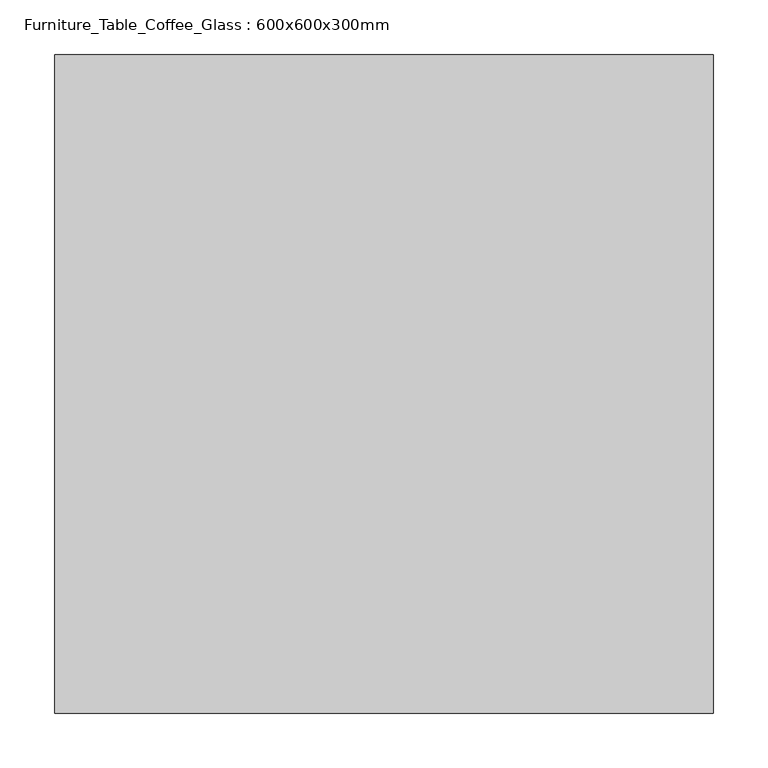
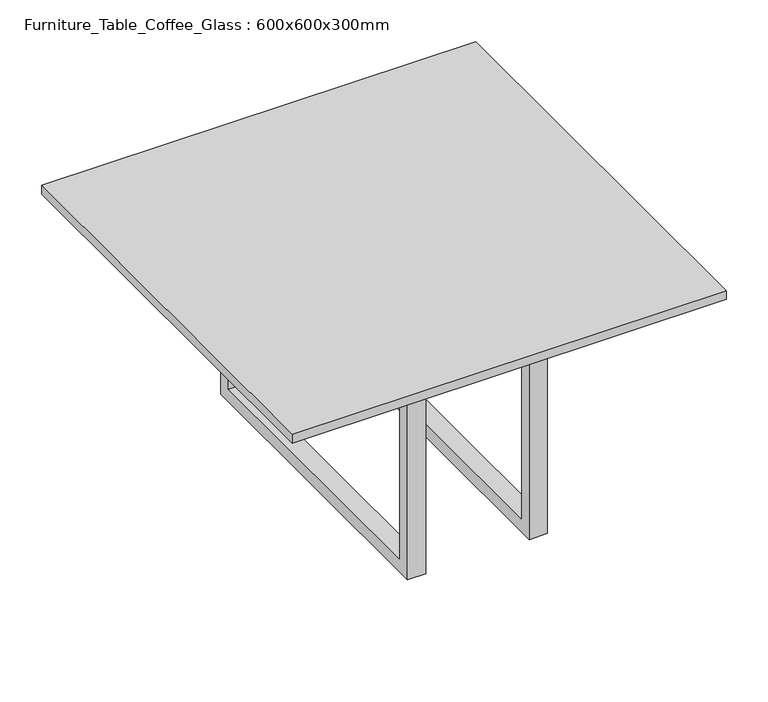
"""IFC4 building model written with IfcOpenShell, lengths in millimetres: furniture geometry, Furniture_Table_Coffee_Glass : 600x600x300mm."""

from ifc_helpers import new_model, si_unit, frame, origin, place, context, project, spatial, polyline, outline, extrude, source, transform, mapped, element, save


def furniture_table_coffee_glass_600x600x300mm_1c447c2e(model_context):
    return source(origin(), model_context, "Body", "SweptSolid", [
        extrude(outline(polyline([(375.1336303, 298.1358318), (375.1336303, 279.0858318), (232.3336303, 279.0858318), (232.3336303, 298.1358318), (375.1336303, 298.1358318)])), frame((0.0, 0.0, 298.25), z_axis=(0.0, 0.0, 1.0), x_axis=(1.0, 0.0, 0.0)), (0.0, 0.0, 1.0), 19.05),
        extrude(outline(polyline([(64.8108318, 317.3), (512.4108318, 317.3), (512.4108318, 0.0), (64.8108318, 0.0), (64.8108318, 317.3)]), holes=[polyline([(83.8608318, 298.25), (83.8608318, 19.05), (493.3608318, 19.05), (493.3608318, 298.25), (83.8608318, 298.25)])]), frame((375.1336303, 0.0, 0.0), z_axis=(1.0, 0.0, 0.0), x_axis=(0.0, 1.0, 0.0)), (0.0, 0.0, 1.0), 25.4),
        extrude(outline(polyline([(64.8108318, 317.3), (512.4108318, 317.3), (512.4108318, 0.0), (64.8108318, 0.0), (64.8108318, 317.3)]), holes=[polyline([(83.8608318, 298.25), (83.8608318, 19.05), (493.3608318, 19.05), (493.3608318, 298.25), (83.8608318, 298.25)])]), frame((206.9336303, 0.0, 0.0), z_axis=(1.0, 0.0, 0.0), x_axis=(0.0, 1.0, 0.0)), (0.0, 0.0, 1.0), 25.4),
        extrude(outline(polyline([(603.7336303, 588.6108318), (603.7336303, -11.3891682), (3.7336303, -11.3891682), (3.7336303, 588.6108318), (603.7336303, 588.6108318)])), frame((0.0, 0.0, 317.3), z_axis=(0.0, 0.0, 1.0), x_axis=(1.0, 0.0, 0.0)), (0.0, 0.0, 1.0), 12.7),
    ])


if __name__ == "__main__":
    model = new_model("IFC4")
    model_context = context("Model", 3, world=origin())
    ifc_project = project(units=[si_unit("LENGTHUNIT", "METRE", prefix="MILLI")], contexts=[model_context])
    site = spatial("IfcSite", under=ifc_project)
    building = spatial("IfcBuilding", under=site)
    placement = place(None, origin())
    furniture_table_coffee_glass_600x600x300mm_shape = furniture_table_coffee_glass_600x600x300mm_1c447c2e(model_context)
    element("IfcFurniture", 1, ObjectType="Furniture_Table_Coffee_Glass : 600x600x300mm", at=placement, inside=building, context=model_context, shape_type="MappedRepresentation", body=[
        mapped(furniture_table_coffee_glass_600x600x300mm_shape, transform((0.0, 0.0, 0.0), x_axis=(1.0, 0.0, 0.0), y_axis=(0.0, 1.0, 0.0), z_axis=(0.0, 0.0, 1.0))),
    ])
    save(model, "model.ifc")

# Revit data of these elements
# Project information
#   Project Status = "Project Status"
#   Client Name = "Revit Project"
#   Project Address = "Enter address here"
#   Project Name = "Two Storey Residence"
#   Project Number = "P.01"
# Type "Furniture_Table_Coffee_Glass : 600x600x300mm"
#   Keynote = "N"
#   Height = 330 mm
#   Length = 600 mm
#   Width = 600 mm
#   Material Base = Metal - Chrome
#   Material Top = Glass - Clear, Grey
#   Assembly Code = ""
# Element 1 (IfcFurniture, "Furniture_Table_Coffee_Glass : 600x600x300mm")
#   Materials on its faces: "Metal - Chrome", "Glass - Clear, Grey"
# Materials
#   "Metal - Chrome": class "Metal", colour RGB 206 206 206, transparency 0
#   "Glass - Clear, Grey": class "Glass", colour RGB 252 255 255, transparency 0.64
